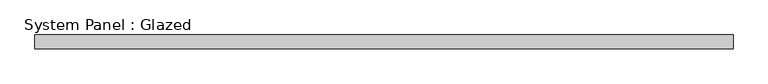
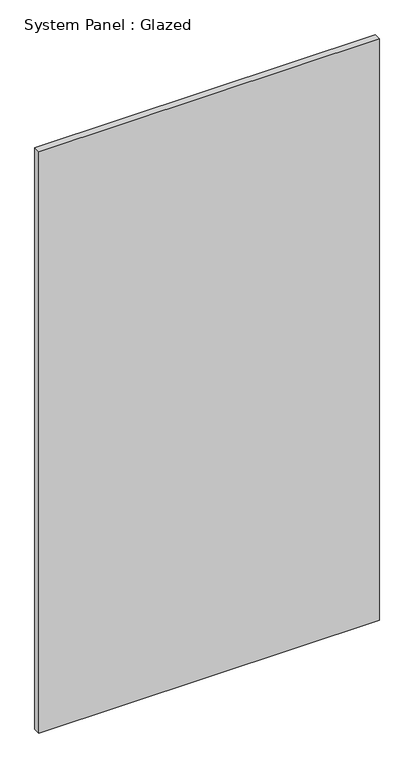
"""IFC4 building model written with IfcOpenShell, lengths in millimetres: plate geometry, System Panel : Glazed."""

from ifc_helpers import new_model, si_unit, origin, origin_with_axes, place, context, project, spatial, polyline, outline, extrude, source, transform, mapped, element, save


def system_panel_glazed_939e179a(model_context):
    return source(origin(), model_context, "Body", "SweptSolid", [
        extrude(outline(polyline([(637.4999999, 24.5), (-637.4999999, 24.5), (-637.4999999, 49.5), (637.4999999, 49.5), (637.4999999, 24.5)])), origin_with_axes(), (0.0, 0.0, 1.0), 2300.0),
    ])


if __name__ == "__main__":
    model = new_model("IFC4")
    model_context = context("Model", 3, world=origin())
    ifc_project = project(units=[si_unit("LENGTHUNIT", "METRE", prefix="MILLI")], contexts=[model_context])
    site = spatial("IfcSite", under=ifc_project)
    building = spatial("IfcBuilding", under=site)
    placement = place(None, origin())
    system_panel_glazed_shape = system_panel_glazed_939e179a(model_context)
    element("IfcPlate", 1, ObjectType="System Panel : Glazed", at=placement, inside=building, context=model_context, shape_type="MappedRepresentation", body=[
        mapped(system_panel_glazed_shape, transform((0.0, 0.0, 0.0), x_axis=(1.0, 0.0, 0.0), y_axis=(0.0, 1.0, 0.0), z_axis=(0.0, 0.0, 1.0))),
    ])
    save(model, "model.ifc")

# Revit data of these elements
# Type "System Panel : Glazed"
#   Construction Type Id = "GSP4R"
#   Analytic Construction = "1/8 in Pilkington single glazing"
#   Visual Light Transmittance = 0.9
#   Solar Heat Gain Coefficient = 0.86
#   Heat Transfer Coefficient (U) = 6.7069 W/(m²·K)
#   Define Thermal Properties by = 1
# Element 1 (IfcPlate, "System Panel : Glazed")
#   Materials on its faces: "Glass"
# Materials
#   "Glass": class "Glass", colour RGB 0 128 192, transparency 0.9, Description = "Soda Lime Glass", Cost = 0
